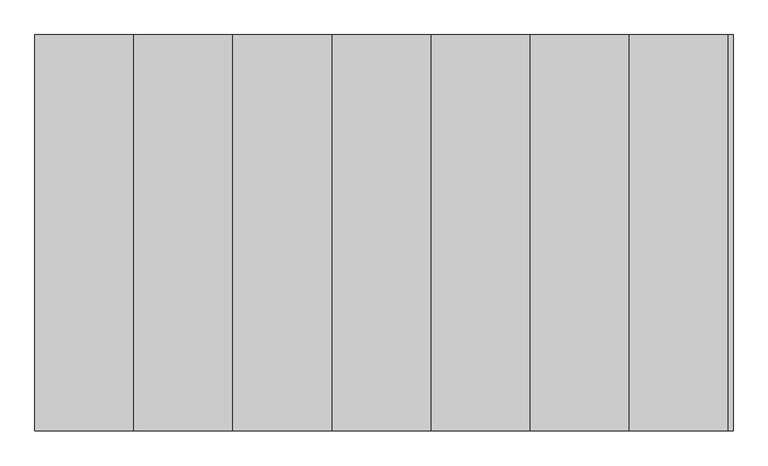
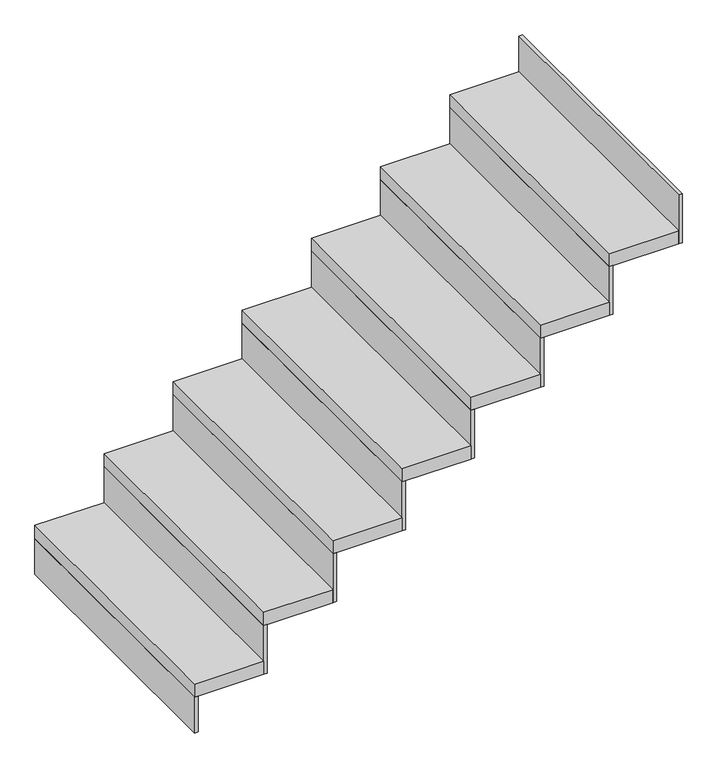
"""IFC4 building model written with IfcOpenShell, lengths in millimetres: stair flight geometry."""

from ifc_helpers import new_model, si_unit, frame, origin, origin_with_axes, place, context, project, spatial, polyline, outline, extrude, source, transform, mapped, element, save


def stair_flight_e7180eca(model_context):
    return source(origin(), model_context, "Body", "SweptSolid", [
        extrude(outline(polyline([(-13562.8533589, -9437.834784), (-13575.3533589, -9437.834784), (-13575.3533589, -8437.834784), (-13562.8533589, -8437.834784), (-13562.8533589, -9437.834784)])), origin_with_axes(), (0.0, 0.0, 1.0), 136.6666667),
        extrude(outline(polyline([(-13325.3533589, -8437.834784), (-13325.3533589, -9437.834784), (-13575.3533589, -9437.834784), (-13575.3533589, -8437.834784), (-13325.3533589, -8437.834784)])), frame((0.0, 0.0, 136.6666667), z_axis=(0.0, 0.0, 1.0), x_axis=(1.0, 0.0, 0.0)), (0.0, 0.0, 1.0), 50.0),
        extrude(outline(polyline([(-13312.8533589, -9437.834784), (-13325.3533589, -9437.834784), (-13325.3533589, -8437.834784), (-13312.8533589, -8437.834784), (-13312.8533589, -9437.834784)])), frame((0.0, 0.0, 136.6666667), z_axis=(0.0, 0.0, 1.0), x_axis=(1.0, 0.0, 0.0)), (0.0, 0.0, 1.0), 186.6666667),
        extrude(outline(polyline([(-13075.3533589, -8437.834784), (-13075.3533589, -9437.834784), (-13325.3533589, -9437.834784), (-13325.3533589, -8437.834784), (-13075.3533589, -8437.834784)])), frame((0.0, 0.0, 323.3333333), z_axis=(0.0, 0.0, 1.0), x_axis=(1.0, 0.0, 0.0)), (0.0, 0.0, 1.0), 50.0),
        extrude(outline(polyline([(-13062.8533589, -9437.834784), (-13075.3533589, -9437.834784), (-13075.3533589, -8437.834784), (-13062.8533589, -8437.834784), (-13062.8533589, -9437.834784)])), frame((0.0, 0.0, 323.3333333), z_axis=(0.0, 0.0, 1.0), x_axis=(1.0, 0.0, 0.0)), (0.0, 0.0, 1.0), 186.6666667),
        extrude(outline(polyline([(-12825.3533589, -8437.834784), (-12825.3533589, -9437.834784), (-13075.3533589, -9437.834784), (-13075.3533589, -8437.834784), (-12825.3533589, -8437.834784)])), frame((0.0, 0.0, 510.0), z_axis=(0.0, 0.0, 1.0), x_axis=(1.0, 0.0, 0.0)), (0.0, 0.0, 1.0), 50.0),
        extrude(outline(polyline([(-12812.8533589, -9437.834784), (-12825.3533589, -9437.834784), (-12825.3533589, -8437.834784), (-12812.8533589, -8437.834784), (-12812.8533589, -9437.834784)])), frame((0.0, 0.0, 510.0), z_axis=(0.0, 0.0, 1.0), x_axis=(1.0, 0.0, 0.0)), (0.0, 0.0, 1.0), 186.6666667),
        extrude(outline(polyline([(-12575.3533589, -8437.834784), (-12575.3533589, -9437.834784), (-12825.3533589, -9437.834784), (-12825.3533589, -8437.834784), (-12575.3533589, -8437.834784)])), frame((0.0, 0.0, 696.6666667), z_axis=(0.0, 0.0, 1.0), x_axis=(1.0, 0.0, 0.0)), (0.0, 0.0, 1.0), 50.0),
        extrude(outline(polyline([(-12562.8533589, -9437.834784), (-12575.3533589, -9437.834784), (-12575.3533589, -8437.834784), (-12562.8533589, -8437.834784), (-12562.8533589, -9437.834784)])), frame((0.0, 0.0, 696.6666667), z_axis=(0.0, 0.0, 1.0), x_axis=(1.0, 0.0, 0.0)), (0.0, 0.0, 1.0), 186.6666667),
        extrude(outline(polyline([(-12325.3533589, -8437.834784), (-12325.3533589, -9437.834784), (-12575.3533589, -9437.834784), (-12575.3533589, -8437.834784), (-12325.3533589, -8437.834784)])), frame((0.0, 0.0, 883.3333333), z_axis=(0.0, 0.0, 1.0), x_axis=(1.0, 0.0, 0.0)), (0.0, 0.0, 1.0), 50.0),
        extrude(outline(polyline([(-12312.8533589, -9437.834784), (-12325.3533589, -9437.834784), (-12325.3533589, -8437.834784), (-12312.8533589, -8437.834784), (-12312.8533589, -9437.834784)])), frame((0.0, 0.0, 883.3333333), z_axis=(0.0, 0.0, 1.0), x_axis=(1.0, 0.0, 0.0)), (0.0, 0.0, 1.0), 186.6666667),
        extrude(outline(polyline([(-12075.3533589, -8437.834784), (-12075.3533589, -9437.834784), (-12325.3533589, -9437.834784), (-12325.3533589, -8437.834784), (-12075.3533589, -8437.834784)])), frame((0.0, 0.0, 1070.0), z_axis=(0.0, 0.0, 1.0), x_axis=(1.0, 0.0, 0.0)), (0.0, 0.0, 1.0), 50.0),
        extrude(outline(polyline([(-12062.8533589, -9437.834784), (-12075.3533589, -9437.834784), (-12075.3533589, -8437.834784), (-12062.8533589, -8437.834784), (-12062.8533589, -9437.834784)])), frame((0.0, 0.0, 1070.0), z_axis=(0.0, 0.0, 1.0), x_axis=(1.0, 0.0, 0.0)), (0.0, 0.0, 1.0), 186.6666667),
        extrude(outline(polyline([(-11825.3533589, -8437.834784), (-11825.3533589, -9437.834784), (-12075.3533589, -9437.834784), (-12075.3533589, -8437.834784), (-11825.3533589, -8437.834784)])), frame((0.0, 0.0, 1256.6666667), z_axis=(0.0, 0.0, 1.0), x_axis=(1.0, 0.0, 0.0)), (0.0, 0.0, 1.0), 50.0),
        extrude(outline(polyline([(-11812.8533589, -9437.834784), (-11825.3533589, -9437.834784), (-11825.3533589, -8437.834784), (-11812.8533589, -8437.834784), (-11812.8533589, -9437.834784)])), frame((0.0, 0.0, 1256.6666667), z_axis=(0.0, 0.0, 1.0), x_axis=(1.0, 0.0, 0.0)), (0.0, 0.0, 1.0), 186.6666667),
    ])


if __name__ == "__main__":
    model = new_model("IFC4")
    model_context = context("Model", 3, world=origin())
    ifc_project = project(units=[si_unit("LENGTHUNIT", "METRE", prefix="MILLI")], contexts=[model_context])
    site = spatial("IfcSite", under=ifc_project)
    building = spatial("IfcBuilding", under=site)
    placement = place(None, origin())
    stair_flight_shape = stair_flight_e7180eca(model_context)
    element("IfcStairFlight", 1, at=placement, inside=building, context=model_context, shape_type="MappedRepresentation", body=[
        mapped(stair_flight_shape, transform((0.0, 0.0, 0.0), x_axis=(1.0, 0.0, 0.0), y_axis=(0.0, 1.0, 0.0), z_axis=(0.0, 0.0, 1.0))),
    ])
    save(model, "model.ifc")
